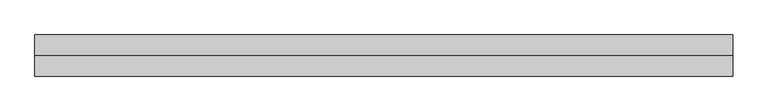
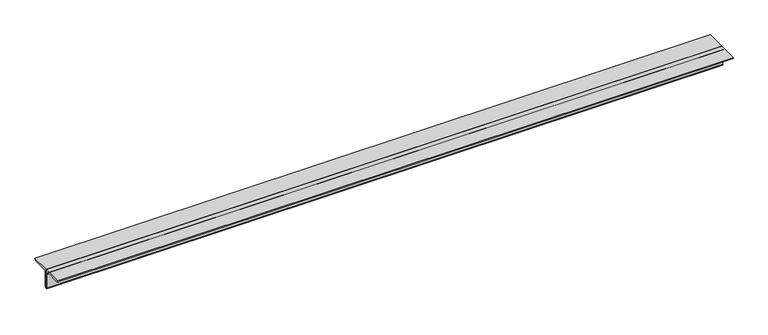
"""IFC4 building model written with IfcOpenShell, lengths in millimetres: member geometry, 0123_Steel Framing_2Ls-KSD3502 : H_SB_AR_S03_2Ls-130x130x12_HBR1."""

from ifc_helpers import new_model, si_unit, point, frame, frame_2d, origin, place, context, project, spatial, polyline, circle_curve, trimmed, segment, composite_curve, outline, extrude, source, transform, mapped, element, save


def member_25707a26(model_context):
    return source(origin(), model_context, "Body", "SweptSolid", [
        extrude(outline(composite_curve([segment(polyline([(0.0, 36.4), (130.0, 36.4)]), True, "CONTINUOUS"), segment(trimmed(circle_curve(frame_2d((118.0, 36.4)), 12.0), [point((130.0, 36.4))], [point((118.0, 24.4))], False, "CARTESIAN"), True, "CONTINUOUS"), segment(polyline([(118.0, 24.4), (24.0, 24.4)]), True, "CONTINUOUS"), segment(trimmed(circle_curve(frame_2d((24.0, 12.4)), 12.0), [point((24.0, 24.4))], [point((12.0, 12.4))], True, "CARTESIAN"), True, "CONTINUOUS"), segment(polyline([(12.0, 12.4), (12.0, -81.6)]), True, "CONTINUOUS"), segment(trimmed(circle_curve(frame_2d((0.0, -81.6)), 12.0), [point((12.0, -81.6))], [point((0.0, -93.6))], False, "CARTESIAN"), True, "CONTINUOUS"), segment(polyline([(0.0, -93.6), (0.0, 36.4)]), True, "CONTINUOUS")], self_intersect=False)), frame((-2254.4342987, 0.0, 0.0), z_axis=(1.0, 0.0, 0.0), x_axis=(0.0, 1.0, 0.0)), (0.0, 0.0, 1.0), 4412.2019305),
        extrude(outline(composite_curve([segment(polyline([(0.0, 36.4), (0.0, -93.6)]), True, "CONTINUOUS"), segment(trimmed(circle_curve(frame_2d((0.0, -81.6)), 12.0), [point((0.0, -93.6))], [point((-12.0, -81.6))], False, "CARTESIAN"), True, "CONTINUOUS"), segment(polyline([(-12.0, -81.6), (-12.0, 12.4)]), True, "CONTINUOUS"), segment(trimmed(circle_curve(frame_2d((-24.0, 12.4)), 12.0), [point((-12.0, 12.4))], [point((-24.0, 24.4))], True, "CARTESIAN"), True, "CONTINUOUS"), segment(polyline([(-24.0, 24.4), (-118.0, 24.4)]), True, "CONTINUOUS"), segment(trimmed(circle_curve(frame_2d((-118.0, 36.4)), 12.0), [point((-118.0, 24.4))], [point((-130.0, 36.4))], False, "CARTESIAN"), True, "CONTINUOUS"), segment(polyline([(-130.0, 36.4), (0.0, 36.4)]), True, "CONTINUOUS")], self_intersect=False)), frame((-2254.4342987, 0.0, 0.0), z_axis=(1.0, 0.0, 0.0), x_axis=(0.0, 1.0, 0.0)), (0.0, 0.0, 1.0), 4412.2019305),
    ])


if __name__ == "__main__":
    model = new_model("IFC4")
    model_context = context("Model", 3, world=origin())
    ifc_project = project(units=[si_unit("LENGTHUNIT", "METRE", prefix="MILLI")], contexts=[model_context])
    site = spatial("IfcSite", under=ifc_project)
    building = spatial("IfcBuilding", under=site)
    placement = place(None, origin())
    member_shape = member_25707a26(model_context)
    element("IfcMember", 1, ObjectType="0123_Steel Framing_2Ls-KSD3502 : H_SB_AR_S03_2Ls-130x130x12_HBR1", at=placement, inside=building, context=model_context, shape_type="MappedRepresentation", body=[
        mapped(member_shape, transform((0.0, 0.0, 0.0), x_axis=(1.0, 0.0, 0.0), y_axis=(0.0, 1.0, 0.0), z_axis=(0.0, 0.0, 1.0))),
    ])
    save(model, "model.ifc")

# Revit data of these elements
# Type "0123_Steel Framing_2Ls-KSD3502 : H_SB_AR_S03_2Ls-130x130x12_HBR1"
#   Type Mark = "HBR1"
#   Assembly Code = "B10"
#   Legs = "SLBB"
#   W = 8.97
#   Perimeter = 1.04 m²/m
#   Nominal Weight = 46.80 kgf/m
#   Length [instance default] = 1000 mm
#   Space = 0 mm
#   b = 130 mm
#   d = 130 mm
#   t = 12 mm
#   y = 36.4 mm
#   A = 0.005952 m²
#   Structural Material [instance default] = Steel ASTM A36
# Element 1 (IfcMember, "0123_Steel Framing_2Ls-KSD3502 : H_SB_AR_S03_2Ls-130x130x12_HBR1")
#   Materials on its faces: "Steel ASTM A36"
# Materials
#   "Steel ASTM A36": class "Metal", colour RGB 199 199 199, transparency 0, Description = "Structural steel, ASTM A36 Grade B, mill finish", Cost = 0
